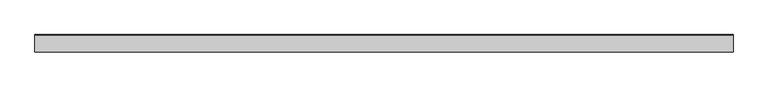
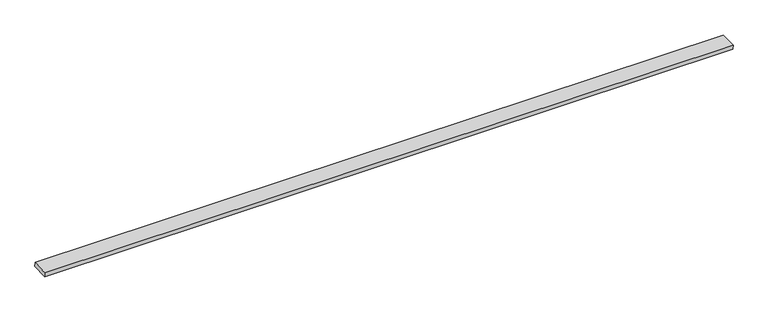
"""IFC4 building model written with IfcOpenShell, lengths in millimetres: proxy geometry, Inner panel:Inner panel:1:Inner panel:1 : Inner panel:Inner panel:300324:2:Inner panel:1:Inner panel:1 : Inner panel:Inner panel:300324:2 : Inner panel:Inner panel:1:Inner panel:1 : Inner panel:Inner panel:300324:300043:21 : Inner panel:Inner panel:1:Inner panel:1 : Inner panel:Inner panel:300324:2:Inner panel:1:Inner panel:1 : Inner panel:Inner panel:300324:2 : Inner panel:Inner panel:1:Inner panel:1 : Inner panel:Inner panel:300324:300043:308120."""

from ifc_helpers import new_model, si_unit, frame, origin, place, context, project, spatial, polyline, outline, extrude, source, transform, mapped, element, save


def generic_models_7b9a4bd1(model_context):
    return source(origin(), model_context, "Body", "SweptSolid", [
        extrude(outline(polyline([(0.0, -119.7013735), (0.0, 0.0), (4876.8, 0.0), (4876.8, -119.7013735), (0.0, -119.7013735)])), frame((596182.8367242, -564831.8307504, 8913.1003942), z_axis=(0.0, -0.041630544712169294, 0.9991330730923526), x_axis=(-1.0, 0.0, 0.0)), (0.0, 0.0, 1.0), 30.353),
    ])


if __name__ == "__main__":
    model = new_model("IFC4")
    model_context = context("Model", 3, world=origin())
    ifc_project = project(units=[si_unit("LENGTHUNIT", "METRE", prefix="MILLI")], contexts=[model_context])
    site = spatial("IfcSite", under=ifc_project)
    building = spatial("IfcBuilding", under=site)
    placement = place(None, origin())
    generic_models_shape = generic_models_7b9a4bd1(model_context)
    element("IfcBuildingElementProxy", 1, Name="Inner panel:Inner panel:1:Inner panel:1 : Inner panel:Inner panel:300324:2:Inner panel:1:Inner panel:1 : Inner panel:Inner panel:300324:2 : Inner panel:Inner panel:1:Inner panel:1 : Inner panel:Inner panel:300324:300043:21 : Inner panel:Inner panel:1:Inner panel:1 : Inner panel:Inner panel:300324:2:Inner panel:1:Inner panel:1 : Inner panel:Inner panel:300324:2 : Inner panel:Inner panel:1:Inner panel:1 : Inner panel:Inner panel:300324:300043:308120", ObjectType="Inner panel:Inner panel:1:Inner panel:1 : Inner panel:Inner panel:300324:2:Inner panel:1:Inner panel:1 : Inner panel:Inner panel:300324:2 : Inner panel:Inner panel:1:Inner panel:1 : Inner panel:Inner panel:300324:300043:21 : Inner panel:Inner panel:1:Inner panel:1 : Inner panel:Inner panel:300324:2:Inner panel:1:Inner panel:1 : Inner panel:Inner panel:300324:2 : Inner panel:Inner panel:1:Inner panel:1 : Inner panel:Inner panel:300324:300043:308120", at=placement, inside=building, context=model_context, shape_type="MappedRepresentation", body=[
        mapped(generic_models_shape, transform((0.0, 0.0, 0.0), x_axis=(1.0, 0.0, 0.0), y_axis=(0.0, 1.0, 0.0), z_axis=(0.0, 0.0, 1.0))),
    ])
    save(model, "model.ifc")

# Revit data of these elements
# Type "Inner panel:Inner panel:1:Inner panel:1 : Inner panel:Inner panel:300324:2:Inner panel:1:Inner panel:1 : Inner panel:Inner panel:300324:2 : Inner panel:Inner panel:1:Inner panel:1 : Inner panel:Inner panel:300324:300043:21 : Inner panel:Inner panel:1:Inner panel:1 : Inner panel:Inner panel:300324:2:Inner panel:1:Inner panel:1 : Inner panel:Inner panel:300324:2 : Inner panel:Inner panel:1:Inner panel:1 : Inner panel:Inner panel:300324:300043:308120"
#   NameOverride = "Inner panel:Inner panel:1:Inner panel:1 : Inner panel:Inner panel:300324:2:Inner panel:1:Inner panel:1 : Inner panel:Inner panel:300324:2 : Inner panel:Inner panel:1:Inner panel:1 : Inner panel:Inner panel:300324:300043:308120"
#   ObjectTypeOverride = "Inner panel:1:Inner panel:1 : Inner panel:Inner panel:300324:2 : Inner panel:Inner panel:1:Inner panel:1 : Inner panel:Inner panel:300324:300043"
#   Reference = "Inner panel"
#   Tag = "308120"
# Element 1 (IfcBuildingElementProxy, "Inner panel:Inner panel:1:Inner panel:1 : Inner panel:Inner panel:300324:2:Inner panel:1:Inner panel:1 : Inner panel:Inner panel:300324:2 : Inner panel:Inner panel:1:Inner panel:1 : Inner panel:Inner panel:300324:300043:21 : Inner panel:Inner panel:1:Inner panel:1 : Inner panel:Inner panel:300324:2:Inner panel:1:Inner panel:1 : Inner panel:Inner panel:300324:2 : Inner panel:Inner panel:1:Inner panel:1 : Inner panel:Inner panel:300324:300043:308120")
#   Materials on its faces: "1\" THERMAL SPACER @ PURLIN"
# Materials
#   "1\" THERMAL SPACER @ PURLIN": class "Unassigned", colour RGB 205 188 106, transparency 0, Cost = 0
